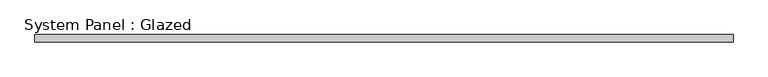
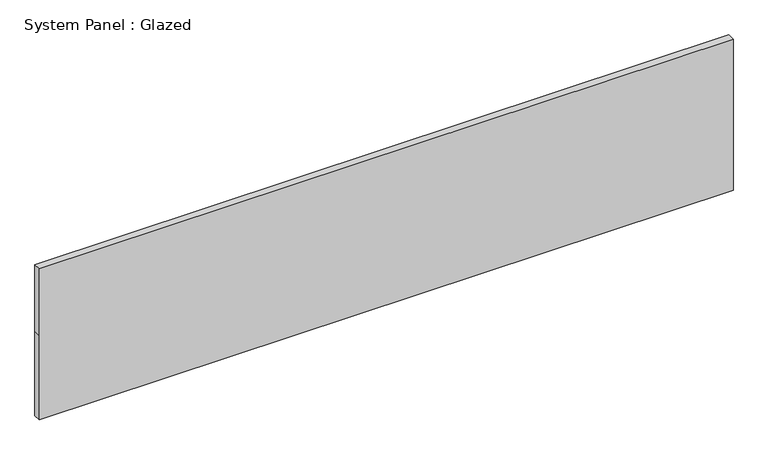
"""IFC4 building model written with IfcOpenShell, lengths in millimetres: plate geometry, System Panel : Glazed."""

from ifc_helpers import new_model, si_unit, frame, origin, place, context, project, spatial, polyline, outline, extrude, source, transform, mapped, element, save


def system_panel_glazed_75890ef7(model_context):
    return source(origin(), model_context, "Body", "SweptSolid", [
        extrude(outline(polyline([(0.0, -1187.45), (0.0, 1187.45), (304.8, 1187.45), (546.1, 1187.45), (546.1, -1187.45), (304.8, -1187.45), (0.0, -1187.45)])), frame((0.0, -44.45, 0.0), z_axis=(0.0, 1.0, 0.0), x_axis=(0.0, 0.0, 1.0)), (0.0, 0.0, 1.0), 25.4),
    ])


if __name__ == "__main__":
    model = new_model("IFC4")
    model_context = context("Model", 3, world=origin())
    ifc_project = project(units=[si_unit("LENGTHUNIT", "METRE", prefix="MILLI")], contexts=[model_context])
    site = spatial("IfcSite", under=ifc_project)
    building = spatial("IfcBuilding", under=site)
    placement = place(None, origin())
    system_panel_glazed_shape = system_panel_glazed_75890ef7(model_context)
    element("IfcPlate", 1, ObjectType="System Panel : Glazed", at=placement, inside=building, context=model_context, shape_type="MappedRepresentation", body=[
        mapped(system_panel_glazed_shape, transform((0.0, 0.0, 0.0), x_axis=(1.0, 0.0, 0.0), y_axis=(0.0, 1.0, 0.0), z_axis=(0.0, 0.0, 1.0))),
    ])
    save(model, "model.ifc")

# Revit data of these elements
# Element 1 (IfcPlate, "System Panel : Glazed")
#   Materials on its faces: "Glass"
# Materials
#   "Glass": class "Glass", colour RGB 0 128 192, transparency 0.75, Cost = 0
